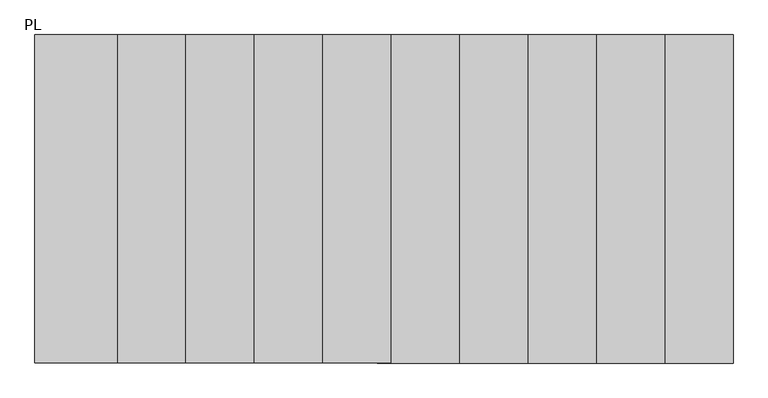
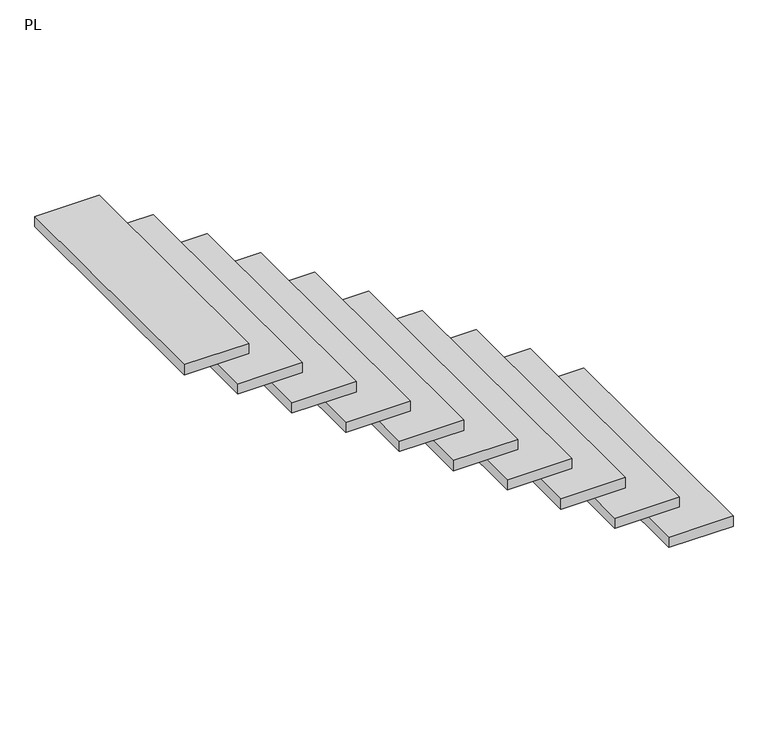
"""IFC4 building model written with IfcOpenShell, lengths in millimetres: stair flight geometry, PL."""

from ifc_helpers import new_model, si_unit, frame, origin, place, context, project, spatial, polyline, outline, extrude, source, transform, mapped, element, save


def pl_11391cdb(model_context):
    return source(origin(), model_context, "Body", "SweptSolid", [
        extrude(outline(polyline([(6009.5374538, 38624.5208589), (6309.5374538, 38624.5208589), (6309.5374538, 37424.5208589), (6009.5374538, 37424.5208589), (6009.5374538, 38624.5208589)])), frame((0.0, 0.0, 731.7901873), z_axis=(0.0, 0.0, 1.0), x_axis=(1.0, 0.0, 0.0)), (0.0, 0.0, 1.0), 50.0),
        extrude(outline(polyline([(5759.5374538, 38624.5208589), (6059.5374538, 38624.5208589), (6059.5374538, 37424.5208589), (5759.5374538, 37424.5208589), (5759.5374538, 38624.5208589)])), frame((0.0, 0.0, 913.6083692), z_axis=(0.0, 0.0, 1.0), x_axis=(1.0, 0.0, 0.0)), (0.0, 0.0, 1.0), 50.0),
        extrude(outline(polyline([(5509.5374538, 38624.5208589), (5809.5374538, 38624.5208589), (5809.5374538, 37424.5208589), (5509.5374538, 37424.5208589), (5509.5374538, 38624.5208589)])), frame((0.0, 0.0, 1095.426551), z_axis=(0.0, 0.0, 1.0), x_axis=(1.0, 0.0, 0.0)), (0.0, 0.0, 1.0), 50.0),
        extrude(outline(polyline([(5259.5374538, 38624.5208589), (5559.5374538, 38624.5208589), (5559.5374538, 37424.5208589), (5259.5374538, 37424.5208589), (5259.5374538, 38624.5208589)])), frame((0.0, 0.0, 1277.2447328), z_axis=(0.0, 0.0, 1.0), x_axis=(1.0, 0.0, 0.0)), (0.0, 0.0, 1.0), 50.0),
        extrude(outline(polyline([(5009.5374538, 38624.5208589), (5309.5374538, 38624.5208589), (5309.5374538, 37424.5208589), (5009.5374538, 37424.5208589), (5009.5374538, 38624.5208589)])), frame((0.0, 0.0, 1459.0629146), z_axis=(0.0, 0.0, 1.0), x_axis=(1.0, 0.0, 0.0)), (0.0, 0.0, 1.0), 50.0),
        extrude(outline(polyline([(4759.5374538, 38624.5208589), (5059.5374538, 38624.5208589), (5059.5374538, 37424.5208589), (4759.5374538, 37424.5208589), (4759.5374538, 38624.5208589)])), frame((0.0, 0.0, 1640.8810964), z_axis=(0.0, 0.0, 1.0), x_axis=(1.0, 0.0, 0.0)), (0.0, 0.0, 1.0), 50.0),
        extrude(outline(polyline([(4509.5374538, 38624.5208589), (4809.5374538, 38624.5208589), (4809.5374538, 37424.5208589), (4509.5374538, 37424.5208589), (4509.5374538, 38624.5208589)])), frame((0.0, 0.0, 1822.6992783), z_axis=(0.0, 0.0, 1.0), x_axis=(1.0, 0.0, 0.0)), (0.0, 0.0, 1.0), 50.0),
        extrude(outline(polyline([(4259.5374538, 38624.5208589), (4559.5374538, 38624.5208589), (4559.5374538, 37424.5208589), (4259.5374538, 37424.5208589), (4259.5374538, 38624.5208589)])), frame((0.0, 0.0, 2004.5174601), z_axis=(0.0, 0.0, 1.0), x_axis=(1.0, 0.0, 0.0)), (0.0, 0.0, 1.0), 50.0),
        extrude(outline(polyline([(4009.5374538, 38624.5208589), (4309.5374538, 38624.5208589), (4309.5374538, 37424.5208589), (4009.5374538, 37424.5208589), (4009.5374538, 38624.5208589)])), frame((0.0, 0.0, 2186.3356419), z_axis=(0.0, 0.0, 1.0), x_axis=(1.0, 0.0, 0.0)), (0.0, 0.0, 1.0), 50.0),
        extrude(outline(polyline([(3759.5374538, 38624.5208589), (4059.5374538, 38624.5208589), (4059.5374538, 37424.5208589), (3759.5374538, 37424.5208589), (3759.5374538, 38624.5208589)])), frame((0.0, 0.0, 2368.1538237), z_axis=(0.0, 0.0, 1.0), x_axis=(1.0, 0.0, 0.0)), (0.0, 0.0, 1.0), 50.0),
    ])


if __name__ == "__main__":
    model = new_model("IFC4")
    model_context = context("Model", 3, world=origin())
    ifc_project = project(units=[si_unit("LENGTHUNIT", "METRE", prefix="MILLI")], contexts=[model_context])
    site = spatial("IfcSite", under=ifc_project)
    building = spatial("IfcBuilding", under=site)
    placement = place(None, origin())
    pl_shape = pl_11391cdb(model_context)
    element("IfcStairFlight", 1, ObjectType="PL", at=placement, inside=building, context=model_context, shape_type="MappedRepresentation", body=[
        mapped(pl_shape, transform((0.0, 0.0, 0.0), x_axis=(1.0, 0.0, 0.0), y_axis=(0.0, 1.0, 0.0), z_axis=(0.0, 0.0, 1.0))),
    ])
    save(model, "model.ifc")
